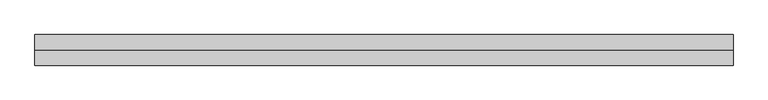
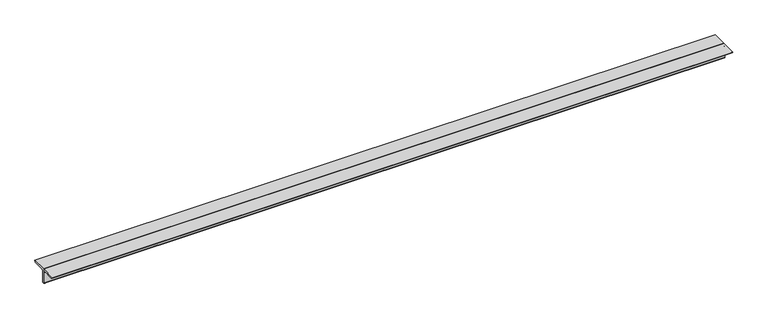
"""IFC4 building model written with IfcOpenShell, lengths in millimetres: member geometry, 0123_Steel Framing_2Ls-KSD3502 : H_SB_AR_S03_2Ls-130x130x12_HBR1."""

import ifcopenshell
import ifcopenshell.guid

model = None  # the IFC model being written
_history = None  # IfcOwnerHistory: only IFC2X3 demands one
_inside = {}  # id of a spatial element -> (the spatial element, [elements in it])
_under = {}  # id of a project, library or spatial element -> (it, [spatial elements below it])
_declared = {}  # id of a project -> (the project, [libraries it declares])
_typed = {}  # id of a type object -> (the type object, [elements of that type])
_made_of = {}  # id of a material, layer set ... -> (it, [elements and type objects made of it])


def new_model(schema):
    """Start an empty IFC model of exactly this schema.

    Asked for "IFC4X3", IfcOpenShell would pick the latest addendum, in which some entities
    have other attributes; the version numbers below select the first issue.
    IFC2X3 requires an IfcOwnerHistory on every rooted entity: one is made here for all.
    """
    global model, _history
    if schema == "IFC4X3":
        model = ifcopenshell.file(schema_version=(4, 3, 0, 0))
    else:
        model = ifcopenshell.file(schema=schema)
    _inside.clear()
    _under.clear()
    _declared.clear()
    _typed.clear()
    _made_of.clear()
    _history = None
    if model.schema == "IFC2X3":
        org = make("IfcOrganization", Name="unknown")
        user = make(
            "IfcPersonAndOrganization",
            ThePerson=make("IfcPerson", FamilyName="unknown"),
            TheOrganization=org,
        )
        app = make(
            "IfcApplication",
            ApplicationDeveloper=org,
            Version="unknown",
            ApplicationFullName="unknown",
            ApplicationIdentifier="unknown",
        )
        _history = make(
            "IfcOwnerHistory",
            OwningUser=user,
            OwningApplication=app,
            ChangeAction="ADDED",
            CreationDate=0,
        )
    return model


def make(cls, **values):
    """One entity of the class cls with the attributes given. An attribute that is None is left unset."""
    return model.create_entity(
        cls, **{name: value for name, value in values.items() if value is not None}
    )


def rooted(cls, **values):
    """An entity with a GlobalId (a new one), such as an element, a storey or a relation."""
    return make(cls, GlobalId=ifcopenshell.guid.new(), OwnerHistory=_history, **values)


def si_unit(unit_type, name, prefix=None):
    """IfcSIUnit, for example si_unit("LENGTHUNIT", "METRE", prefix="MILLI")."""
    return make("IfcSIUnit", UnitType=unit_type, Prefix=prefix, Name=name)


def assignment(units):
    """IfcUnitAssignment: the units of a project."""
    return None if units is None else make("IfcUnitAssignment", Units=units)


def point(xyz):
    """IfcCartesianPoint."""
    return None if xyz is None else make("IfcCartesianPoint", Coordinates=xyz)


def direction(xyz):
    """IfcDirection."""
    return None if xyz is None else make("IfcDirection", DirectionRatios=xyz)


def frame(location, z_axis=None, x_axis=None):
    """IfcAxis2Placement3D, a coordinate frame: its origin and axes. An axis left out is left unset."""
    return make(
        "IfcAxis2Placement3D",
        Location=point(location),
        Axis=direction(z_axis),
        RefDirection=direction(x_axis),
    )


def frame_2d(location, x_axis=None):
    """IfcAxis2Placement2D, a coordinate frame in the plane: its origin and x axis."""
    return make(
        "IfcAxis2Placement2D", Location=point(location), RefDirection=direction(x_axis)
    )


def origin():
    """The frame at (0, 0, 0) with its axes left unset."""
    return frame((0.0, 0.0, 0.0))


def place(relative_to, where):
    """IfcLocalPlacement: puts the frame where relative to a parent placement (None: the world)."""
    return make(
        "IfcLocalPlacement", PlacementRelTo=relative_to, RelativePlacement=where
    )


def context(
    kind, dimensions, precision=None, world=None, true_north=None, identifier=None
):
    """IfcGeometricRepresentationContext, for example the 3D "Model" context."""
    return make(
        "IfcGeometricRepresentationContext",
        ContextIdentifier=identifier,
        ContextType=kind,
        CoordinateSpaceDimension=dimensions,
        Precision=precision,
        WorldCoordinateSystem=world,
        TrueNorth=true_north,
    )


def project(units=None, contexts=None):
    """IfcProject with its units and contexts."""
    return rooted(
        "IfcProject",
        Name="project",
        RepresentationContexts=contexts,
        UnitsInContext=assignment(units),
    )


def spatial(cls, under=None, at=None, **own):
    """A site, building, storey or space (cls), placed at a placement, below another one or the project."""
    s = rooted(cls, ObjectPlacement=at, **own)
    if under is not None:
        _under.setdefault(under.id(), (under, []))[1].append(s)
    return s


def polyline(points):
    """IfcPolyline through the points."""
    return make("IfcPolyline", Points=[point(p) for p in points])


def circle_curve(where, radius):
    """IfcCircle in the frame where."""
    return make("IfcCircle", Position=where, Radius=radius)


def trimmed(basis, trim1, trim2, sense, master):
    """IfcTrimmedCurve: the piece of a basis curve between two trims."""
    return make(
        "IfcTrimmedCurve",
        BasisCurve=basis,
        Trim1=trim1,
        Trim2=trim2,
        SenseAgreement=sense,
        MasterRepresentation=master,
    )


def segment(curve, same_sense, transition):
    """IfcCompositeCurveSegment."""
    return make(
        "IfcCompositeCurveSegment",
        Transition=transition,
        SameSense=same_sense,
        ParentCurve=curve,
    )


def composite_curve(segments, self_intersect=None):
    """IfcCompositeCurve: segments joined end to end."""
    return make("IfcCompositeCurve", Segments=segments, SelfIntersect=self_intersect)


def outline(outer, holes=None, kind="AREA"):
    """IfcArbitraryClosedProfileDef: a profile drawn as a closed curve; with holes, ...WithVoids."""
    if holes is None:
        return make("IfcArbitraryClosedProfileDef", ProfileType=kind, OuterCurve=outer)
    return make(
        "IfcArbitraryProfileDefWithVoids",
        ProfileType=kind,
        OuterCurve=outer,
        InnerCurves=holes,
    )


def extrude(swept, where, along, depth):
    """IfcExtrudedAreaSolid: the profile swept, set in the frame where, extruded along a direction by depth."""
    return make(
        "IfcExtrudedAreaSolid",
        SweptArea=swept,
        Position=where,
        ExtrudedDirection=direction(along),
        Depth=depth,
    )


def shape(context_of_items, identifier, shape_type, items):
    """IfcShapeRepresentation: the items that make up one representation, for example the "Body"."""
    return make(
        "IfcShapeRepresentation",
        ContextOfItems=context_of_items,
        RepresentationIdentifier=identifier,
        RepresentationType=shape_type,
        Items=items,
    )


def source(mapping_origin, context_of_items, identifier, shape_type, items):
    """IfcRepresentationMap: a shape defined once, which mapped items show again and again."""
    return make(
        "IfcRepresentationMap",
        MappingOrigin=mapping_origin,
        MappedRepresentation=shape(context_of_items, identifier, shape_type, items),
    )


def transform(
    local_origin,
    x_axis=None,
    y_axis=None,
    z_axis=None,
    scale=None,
    scale2=None,
    scale3=None,
    uniform=True,
):
    """IfcCartesianTransformationOperator3D, or its non-uniform kind. x_axis, y_axis, z_axis: its Axis1, 2, 3."""
    if uniform:
        return make(
            "IfcCartesianTransformationOperator3D",
            Axis1=direction(x_axis),
            Axis2=direction(y_axis),
            LocalOrigin=point(local_origin),
            Scale=scale,
            Axis3=direction(z_axis),
        )
    return make(
        "IfcCartesianTransformationOperator3DnonUniform",
        Axis1=direction(x_axis),
        Axis2=direction(y_axis),
        LocalOrigin=point(local_origin),
        Scale=scale,
        Axis3=direction(z_axis),
        Scale2=scale2,
        Scale3=scale3,
    )


def mapped(mapping_source, mapping_target):
    """IfcMappedItem: shows the shape of a source again, moved by a transform."""
    return make(
        "IfcMappedItem", MappingSource=mapping_source, MappingTarget=mapping_target
    )


def made_of(thing, what):
    """Note that an element or type object is made of a material, layer set ...; save() writes the relation."""
    if what is not None:
        _made_of.setdefault(what.id(), (what, []))[1].append(thing)
    return thing


def element(
    cls,
    number,
    at=None,
    inside=None,
    cuts=None,
    type_object=None,
    material=None,
    context=None,
    identifier="Body",
    shape_type=None,
    held_by="IfcProductDefinitionShape",
    body=None,
    shapes=None,
    **own,
):
    """One element of the class cls, such as IfcWall. Its Tag is "e" and its number.

    at: its placement. inside: the storey or other place that contains it. cuts: it is an
    opening in that element (IfcRelVoidsElement). A single representation is given by context,
    identifier, shape_type and body (its items); several are given by shapes. held_by: the class
    of the entity that holds the representations. save() writes the other relations.
    """
    e = rooted(cls, Tag="e%d" % number, ObjectPlacement=at, **own)
    if body is not None:
        shapes = [shape(context, identifier, shape_type, body)]
    if shapes is not None:
        e.Representation = make(held_by, Representations=shapes)
    if inside is not None:
        _inside.setdefault(inside.id(), (inside, []))[1].append(e)
    if cuts is not None:
        rooted(
            "IfcRelVoidsElement", RelatingBuildingElement=cuts, RelatedOpeningElement=e
        )
    if type_object is not None:
        _typed.setdefault(type_object.id(), (type_object, []))[1].append(e)
    return made_of(e, material)


def aggregate(whole, parts):
    """IfcRelAggregates: a whole, such as a stair, and the parts it consists of."""
    return rooted("IfcRelAggregates", RelatingObject=whole, RelatedObjects=parts)


def save(model, path):
    """Write the relations noted so far, then the file.

    IfcRelAggregates (storeys below a building ...), IfcRelContainedInSpatialStructure (elements
    in a storey), IfcRelDefinesByType, IfcRelAssociatesMaterial and IfcRelDeclares: one each for
    every whole, place, type object, material and project.
    """
    for whole, parts in _under.values():
        aggregate(whole, parts)
    for where, things in _inside.values():
        rooted(
            "IfcRelContainedInSpatialStructure",
            RelatedElements=things,
            RelatingStructure=where,
        )
    for kind, things in _typed.values():
        rooted("IfcRelDefinesByType", RelatedObjects=things, RelatingType=kind)
    for what, things in _made_of.values():
        rooted("IfcRelAssociatesMaterial", RelatedObjects=things, RelatingMaterial=what)
    for by, libraries in _declared.values():
        rooted("IfcRelDeclares", RelatingContext=by, RelatedDefinitions=libraries)
    model.write(path)


def member_e3b25103(model_context):
    return source(origin(), model_context, "Body", "SweptSolid", [
        extrude(outline(composite_curve([segment(polyline([(0.0, 36.4), (130.0, 36.4)]), True, "CONTINUOUS"), segment(trimmed(circle_curve(frame_2d((118.0, 36.4)), 12.0), [point((130.0, 36.4))], [point((118.0, 24.4))], False, "CARTESIAN"), True, "CONTINUOUS"), segment(polyline([(118.0, 24.4), (24.0, 24.4)]), True, "CONTINUOUS"), segment(trimmed(circle_curve(frame_2d((24.0, 12.4)), 12.0), [point((24.0, 24.4))], [point((12.0, 12.4))], True, "CARTESIAN"), True, "CONTINUOUS"), segment(polyline([(12.0, 12.4), (12.0, -81.6)]), True, "CONTINUOUS"), segment(trimmed(circle_curve(frame_2d((0.0, -81.6)), 12.0), [point((12.0, -81.6))], [point((0.0, -93.6))], False, "CARTESIAN"), True, "CONTINUOUS"), segment(polyline([(0.0, -93.6), (0.0, 36.4)]), True, "CONTINUOUS")], self_intersect=False)), frame((-2965.840786, 0.0, 0.0), z_axis=(1.0, 0.0, 0.0), x_axis=(0.0, 1.0, 0.0)), (0.0, 0.0, 1.0), 5929.4021426),
        extrude(outline(composite_curve([segment(polyline([(0.0, 36.4), (0.0, -93.6)]), True, "CONTINUOUS"), segment(trimmed(circle_curve(frame_2d((0.0, -81.6)), 12.0), [point((0.0, -93.6))], [point((-12.0, -81.6))], False, "CARTESIAN"), True, "CONTINUOUS"), segment(polyline([(-12.0, -81.6), (-12.0, 12.4)]), True, "CONTINUOUS"), segment(trimmed(circle_curve(frame_2d((-24.0, 12.4)), 12.0), [point((-12.0, 12.4))], [point((-24.0, 24.4))], True, "CARTESIAN"), True, "CONTINUOUS"), segment(polyline([(-24.0, 24.4), (-118.0, 24.4)]), True, "CONTINUOUS"), segment(trimmed(circle_curve(frame_2d((-118.0, 36.4)), 12.0), [point((-118.0, 24.4))], [point((-130.0, 36.4))], False, "CARTESIAN"), True, "CONTINUOUS"), segment(polyline([(-130.0, 36.4), (0.0, 36.4)]), True, "CONTINUOUS")], self_intersect=False)), frame((-2965.840786, 0.0, 0.0), z_axis=(1.0, 0.0, 0.0), x_axis=(0.0, 1.0, 0.0)), (0.0, 0.0, 1.0), 5929.4021426),
    ])


if __name__ == "__main__":
    model = new_model("IFC4")
    model_context = context("Model", 3, world=origin())
    ifc_project = project(units=[si_unit("LENGTHUNIT", "METRE", prefix="MILLI")], contexts=[model_context])
    site = spatial("IfcSite", under=ifc_project)
    building = spatial("IfcBuilding", under=site)
    placement = place(None, origin())
    member_shape = member_e3b25103(model_context)
    element("IfcMember", 1, ObjectType="0123_Steel Framing_2Ls-KSD3502 : H_SB_AR_S03_2Ls-130x130x12_HBR1", at=placement, inside=building, context=model_context, shape_type="MappedRepresentation", body=[
        mapped(member_shape, transform((0.0, 0.0, 0.0), x_axis=(1.0, 0.0, 0.0), y_axis=(0.0, 1.0, 0.0), z_axis=(0.0, 0.0, 1.0))),
    ])
    save(model, "model.ifc")

# Revit data of these elements
# Type "0123_Steel Framing_2Ls-KSD3502 : H_SB_AR_S03_2Ls-130x130x12_HBR1"
#   Assembly Code = "B10"
#   Legs = "SLBB"
#   W = 8.97
#   Perimeter = 1.04 m²/m
#   Nominal Weight = 46.80 kgf/m
#   Length [instance default] = 1000 mm
#   Space = 0 mm
#   b = 130 mm
#   d = 130 mm
#   t = 12 mm
#   y = 36.4 mm
#   A = 0.005952 m²
#   Structural Material [instance default] = Steel ASTM A36
# Element 1 (IfcMember, "0123_Steel Framing_2Ls-KSD3502 : H_SB_AR_S03_2Ls-130x130x12_HBR1")
#   Structural Material = Steel, 45-345
#   Materials on its faces: "Steel, 45-345"
# Materials
#   "Steel ASTM A36": class "Metal", colour RGB 199 199 199, transparency 0, Description = "Structural steel, ASTM A36 Grade B, mill finish", Cost = 0
#   "Steel, 45-345": class "Metal", colour RGB 189 187 185, transparency 0, Description = "Steel 345 MPa", Cost = 0
